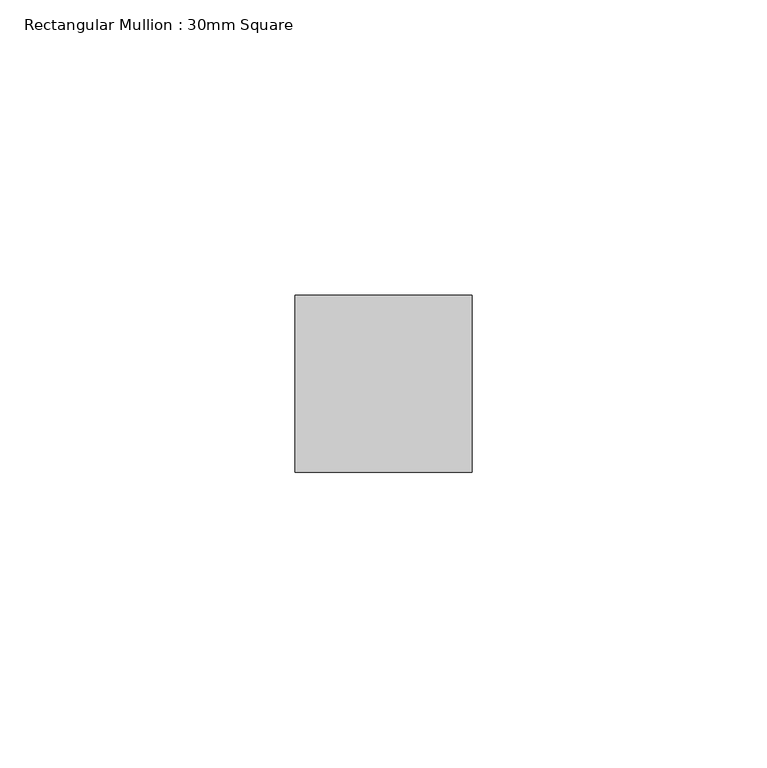
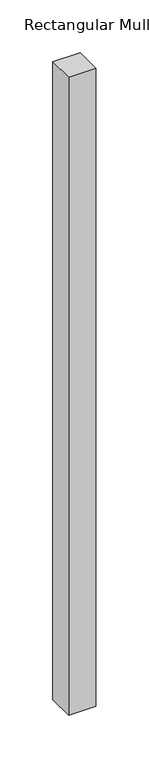
"""IFC4 building model written with IfcOpenShell, lengths in millimetres: member geometry, Rectangular Mullion : 30mm Square."""

from ifc_helpers import new_model, si_unit, frame, origin, place, context, project, spatial, polyline, outline, extrude, source, transform, mapped, element, save


def rectangular_mullion_30mm_square_7ac6073e(model_context):
    return source(origin(), model_context, "Body", "SweptSolid", [
        extrude(outline(polyline([(15.0, 15.0), (15.0, -15.0), (-15.0, -15.0), (-15.0, 15.0), (15.0, 15.0)])), frame((0.0, 0.0, -738.7218892), z_axis=(0.0, 0.0, 1.0), x_axis=(1.0, 0.0, 0.0)), (0.0, 0.0, 1.0), 738.7218892),
    ])


if __name__ == "__main__":
    model = new_model("IFC4")
    model_context = context("Model", 3, world=origin())
    ifc_project = project(units=[si_unit("LENGTHUNIT", "METRE", prefix="MILLI")], contexts=[model_context])
    site = spatial("IfcSite", under=ifc_project)
    building = spatial("IfcBuilding", under=site)
    placement = place(None, origin())
    rectangular_mullion_30mm_square_shape = rectangular_mullion_30mm_square_7ac6073e(model_context)
    element("IfcMember", 1, ObjectType="Rectangular Mullion : 30mm Square", at=placement, inside=building, context=model_context, shape_type="MappedRepresentation", body=[
        mapped(rectangular_mullion_30mm_square_shape, transform((0.0, 0.0, 0.0), x_axis=(1.0, 0.0, 0.0), y_axis=(0.0, 1.0, 0.0), z_axis=(0.0, 0.0, 1.0))),
    ])
    save(model, "model.ifc")

# Revit data of these elements
# Type "Rectangular Mullion : 30mm Square"
#   built-in parameter 1007304 = 0.0984252 (stored number, unit not read)
#   built-in parameter 1007301 = 0.0492126 (stored number, unit not read)
#   built-in parameter 1007300 = 0.0492126 (stored number, unit not read)
# Element 1 (IfcMember, "Rectangular Mullion : 30mm Square")
#   Materials on its faces: "Aluminum"
# Materials
#   "Aluminum": class "Metal", colour RGB 244 244 244, transparency 0, Description = "Aluminum 6061", Cost = 0
